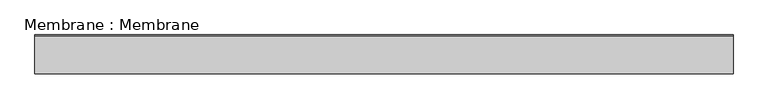
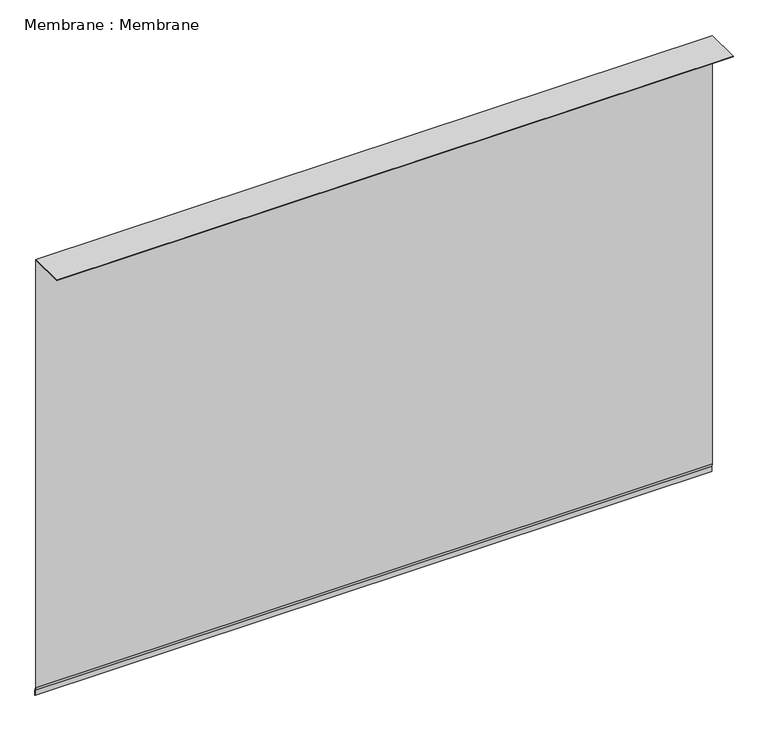
"""IFC4 building model written with IfcOpenShell, lengths in millimetres: proxy geometry, Membrane : Membrane."""

from ifc_helpers import new_model, si_unit, frame, origin, place, context, project, spatial, polyline, outline, extrude, source, transform, mapped, element, save


def membrane_membrane_7833c3fc(model_context):
    return source(origin(), model_context, "Body", "SweptSolid", [
        extrude(outline(polyline([(10332.3117604, 40775.4101563), (10439.111229, 40775.4101563), (10439.111229, 39437.1078269), (10443.1968914, 39425.8825617), (10443.1968914, 39410.30025), (10442.1968914, 39410.30025), (10442.1968914, 39425.7062347), (10438.111229, 39436.9314999), (10438.111229, 40774.4101563), (10332.3117604, 40774.4101563), (10332.3117604, 40775.4101563)])), frame((3694.2883192, 0.0, 0.0), z_axis=(1.0, 0.0, 0.0), x_axis=(0.0, 1.0, 0.0)), (0.0, 0.0, 1.0), 2000.0),
    ])


if __name__ == "__main__":
    model = new_model("IFC4")
    model_context = context("Model", 3, world=origin())
    ifc_project = project(units=[si_unit("LENGTHUNIT", "METRE", prefix="MILLI")], contexts=[model_context])
    site = spatial("IfcSite", under=ifc_project)
    building = spatial("IfcBuilding", under=site)
    placement = place(None, origin())
    membrane_membrane_shape = membrane_membrane_7833c3fc(model_context)
    element("IfcBuildingElementProxy", 1, Name="Membrane : Membrane", ObjectType="Membrane : Membrane", at=placement, inside=building, context=model_context, shape_type="MappedRepresentation", body=[
        mapped(membrane_membrane_shape, transform((0.0, 0.0, 0.0), x_axis=(1.0, 0.0, 0.0), y_axis=(0.0, 1.0, 0.0), z_axis=(0.0, 0.0, 1.0))),
    ])
    save(model, "model.ifc")

# Revit data of these elements
# Type "Membrane : Membrane"
#   NameOverride = "Membrane"
# Element 1 (IfcBuildingElementProxy, "Membrane : Membrane")
#   Materials on its faces: "(2) LAYERS OF ICE AND WATER SHIELD (BITUTHANE) UNDER STUCCO"
# Materials
#   "(2) LAYERS OF ICE AND WATER SHIELD (BITUTHANE) UNDER STUCCO": class "Unassigned", colour RGB 186 255 159, transparency 0, Cost = 0
